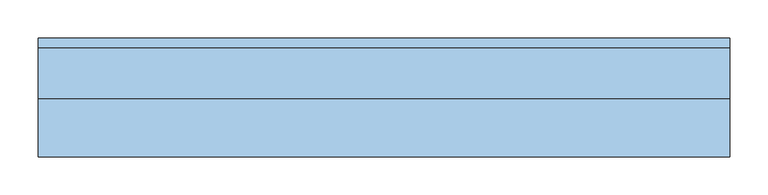
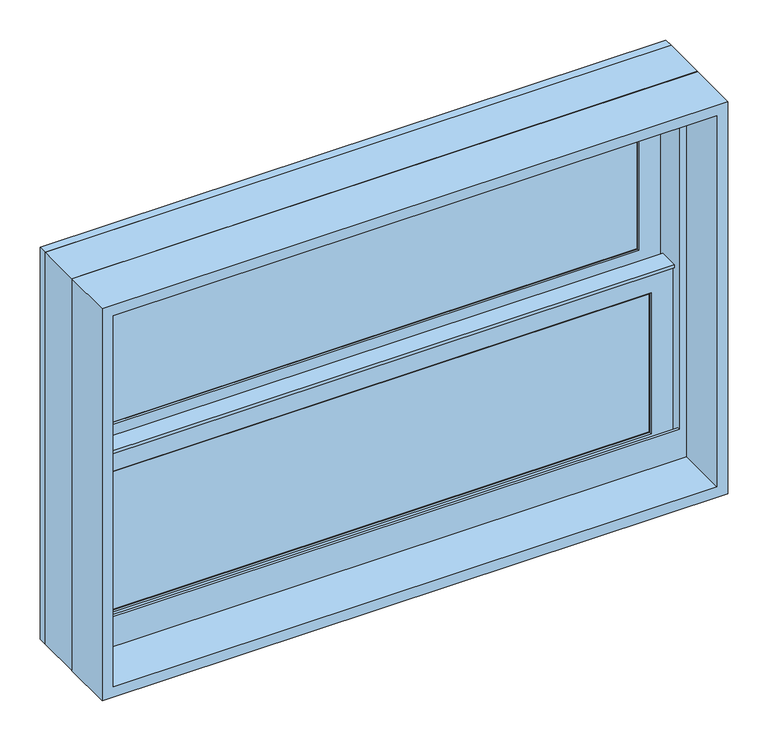
"""IFC4 building model written with IfcOpenShell, lengths in millimetres: window geometry, Window-Double_Hung-Marvin-Essential : ESDH3020."""

from ifc_helpers import new_model, si_unit, frame, origin, place, context, project, spatial, polyline, outline, extrude, faceted_brep, source, transform, mapped, element, save


def window_0800c113(model_context):
    return source(origin(), model_context, "Body", "SolidModel", [
        extrude(outline(polyline([(140.7583333, 20.6375), (140.7583333, 15.875), (121.7083333, 15.875), (121.7083333, 20.6375), (140.7583333, 20.6375)])), frame((0.0, 0.0, 1898.65), z_axis=(0.0, 0.0, 1.0), x_axis=(1.0, 0.0, 0.0)), (0.0, 0.0, 1.0), 222.25),
        extrude(outline(polyline([(-121.7083333, 20.6375), (-121.7083333, 15.875), (-140.7583333, 15.875), (-140.7583333, 20.6375), (-121.7083333, 20.6375)])), frame((0.0, 0.0, 1898.65), z_axis=(0.0, 0.0, 1.0), x_axis=(1.0, 0.0, 0.0)), (0.0, 0.0, 1.0), 222.25),
        extrude(outline(polyline([(393.7, 20.6375), (393.7, 15.875), (-393.7, 15.875), (-393.7, 20.6375), (393.7, 20.6375)])), frame((0.0, 0.0, 2000.25), z_axis=(0.0, 0.0, 1.0), x_axis=(1.0, 0.0, 0.0)), (0.0, 0.0, 1.0), 19.05),
        extrude(outline(polyline([(-140.7583333, 46.83125), (-140.7583333, 51.59375), (-121.7083333, 51.59375), (-121.7083333, 46.83125), (-140.7583333, 46.83125)])), frame((0.0, 0.0, 2159.0), z_axis=(0.0, 0.0, 1.0), x_axis=(1.0, 0.0, 0.0)), (0.0, 0.0, 1.0), 222.25),
        extrude(outline(polyline([(121.7083333, 46.83125), (121.7083333, 51.59375), (140.7583333, 51.59375), (140.7583333, 46.83125), (121.7083333, 46.83125)])), frame((0.0, 0.0, 2159.0), z_axis=(0.0, 0.0, 1.0), x_axis=(1.0, 0.0, 0.0)), (0.0, 0.0, 1.0), 222.25),
        extrude(outline(polyline([(-393.7, 46.83125), (-393.7, 51.59375), (393.7, 51.59375), (393.7, 46.83125), (-393.7, 46.83125)])), frame((0.0, 0.0, 2260.6), z_axis=(0.0, 0.0, 1.0), x_axis=(1.0, 0.0, 0.0)), (0.0, 0.0, 1.0), 19.05),
        extrude(outline(polyline([(140.7583333, 20.6375), (121.7083333, 20.6375), (121.7083333, 25.4), (140.7583333, 25.4), (140.7583333, 20.6375)])), frame((0.0, 0.0, 1898.65), z_axis=(0.0, 0.0, 1.0), x_axis=(1.0, 0.0, 0.0)), (0.0, 0.0, 1.0), 222.25),
        extrude(outline(polyline([(-121.7083333, 20.6375), (-140.7583333, 20.6375), (-140.7583333, 25.4), (-121.7083333, 25.4), (-121.7083333, 20.6375)])), frame((0.0, 0.0, 1898.65), z_axis=(0.0, 0.0, 1.0), x_axis=(1.0, 0.0, 0.0)), (0.0, 0.0, 1.0), 222.25),
        extrude(outline(polyline([(393.7, 20.6375), (-393.7, 20.6375), (-393.7, 25.4), (393.7, 25.4), (393.7, 20.6375)])), frame((0.0, 0.0, 2000.25), z_axis=(0.0, 0.0, 1.0), x_axis=(1.0, 0.0, 0.0)), (0.0, 0.0, 1.0), 19.05),
        extrude(outline(polyline([(-140.7583333, 56.35625), (-121.7083333, 56.35625), (-121.7083333, 51.59375), (-140.7583333, 51.59375), (-140.7583333, 56.35625)])), frame((0.0, 0.0, 2159.0), z_axis=(0.0, 0.0, 1.0), x_axis=(1.0, 0.0, 0.0)), (0.0, 0.0, 1.0), 222.25),
        extrude(outline(polyline([(121.7083333, 56.35625), (140.7583333, 56.35625), (140.7583333, 51.59375), (121.7083333, 51.59375), (121.7083333, 56.35625)])), frame((0.0, 0.0, 2159.0), z_axis=(0.0, 0.0, 1.0), x_axis=(1.0, 0.0, 0.0)), (0.0, 0.0, 1.0), 222.25),
        extrude(outline(polyline([(-393.7, 56.35625), (393.7, 56.35625), (393.7, 51.59375), (-393.7, 51.59375), (-393.7, 56.35625)])), frame((0.0, 0.0, 2260.6), z_axis=(0.0, 0.0, 1.0), x_axis=(1.0, 0.0, 0.0)), (0.0, 0.0, 1.0), 19.05),
        faceted_brep([(-420.6875, 5.6780605, 2150.9351748), (-420.6875, 5.6780605, 2146.3), (420.6875, 5.6780605, 2146.3), (420.6875, 5.6780605, 2150.9351748), (-420.6875, 34.8118605, 2150.9351748), (420.6875, 34.8118605, 2150.9351748), (420.6875, 34.8118605, 2146.3), (-420.6875, 34.8118605, 2146.3), (-420.6875, 30.1625, 2146.3), (-420.6875, 30.1625, 1871.6625), (-420.6875, 8.9241104, 1871.6625), (-420.6875, 8.9241104, 2146.3), (420.6875, 8.9241104, 2146.3), (420.6875, 30.1625, 2146.3), (420.6875, 8.9241104, 1871.6625), (420.6875, 30.1625, 1871.6625), (-404.8034752, 11.90625, 2132.0034752), (-404.8034752, 30.1625, 2132.0034752), (404.8034752, 30.1625, 2132.0034752), (404.8034752, 11.90625, 2132.0034752), (-388.14375, 10.4662439, 2115.34375), (-388.14375, 11.90625, 2115.34375), (388.14375, 11.90625, 2115.34375), (388.14375, 10.4662439, 2115.34375), (389.6858834, 8.9241104, 2116.8858834), (-389.6858834, 8.9241104, 2116.8858834), (404.8034752, 30.1625, 1887.5465248), (404.8034752, 11.90625, 1887.5465248), (388.14375, 11.90625, 1904.20625), (388.14375, 10.4662439, 1904.20625), (389.6858834, 8.9241104, 1902.6641166), (-404.8034752, 30.1625, 1887.5465248), (-404.8034752, 11.90625, 1887.5465248), (-388.14375, 11.90625, 1904.20625), (-388.14375, 10.4662439, 1904.20625), (-389.6858834, 8.9241104, 1902.6641166)], [[[0, 1, 2, 3]], [[4, 5, 6, 7]], [[1, 0, 4, 7, 8, 9, 10, 11]], [[2, 1, 11, 12]], [[7, 6, 13, 8]], [[3, 2, 12, 14, 15, 13, 6, 5]], [[0, 3, 5, 4]], [[16, 17, 18, 19]], [[20, 21, 22, 23]], [[20, 23, 24, 25]], [[19, 18, 26, 27]], [[23, 22, 28, 29]], [[24, 23, 29, 30]], [[27, 26, 31, 32]], [[29, 28, 33, 34]], [[30, 29, 34, 35]], [[15, 14, 10, 9]], [[15, 9, 8, 13], [18, 17, 31, 26]], [[17, 16, 32, 31]], [[16, 19, 27, 32], [22, 21, 33, 28]], [[21, 20, 34, 33]], [[20, 25, 35, 34]], [[10, 14, 12, 11], [25, 24, 30, 35]]]),
        extrude(outline(polyline([(38.5955581, 2132.0125), (33.5778968, 2132.0125), (33.5778968, 2133.6), (39.9405976, 2133.6), (39.9405976, 2132.0125), (61.515625, 2132.0125), (47.6307501, 2128.6975159), (38.5955581, 2128.6975159), (38.5955581, 2132.0125)])), frame((-420.6875, 0.0, 0.0), z_axis=(1.0, 0.0, 0.0), x_axis=(0.0, 1.0, 0.0)), (0.0, 0.0, 1.0), 841.375),
        faceted_brep([(450.85, 0.0, 1841.5), (450.85, 0.0, 2438.4), (-450.85, 0.0, 2438.4), (-450.85, 0.0, 1841.5), (424.65625, 0.0, 1902.61875), (-424.65625, 0.0, 1902.61875), (-424.65625, 0.0, 2412.20625), (424.65625, 0.0, 2412.20625), (424.65625, 3.96875, 1841.5), (-424.65625, 3.96875, 1841.5), (-424.65625, 3.96875, 1902.61875), (424.65625, 3.96875, 1902.61875), (-450.85, 65.6828125, 1841.5), (-424.65625, 65.6828125, 1841.5), (424.65625, 65.6828125, 1841.5), (450.85, 65.6828125, 1841.5), (-450.85, 65.6828125, 2438.4), (450.85, 65.6828125, 2438.4), (424.65625, 65.6828125, 2412.20625), (-424.65625, 65.6828125, 2412.20625)], [[[0, 1, 2, 3], [4, 5, 6, 7]], [[8, 9, 10, 11]], [[5, 4, 11, 10]], [[0, 3, 12, 13, 9, 8, 14, 15]], [[13, 12, 16, 17, 15, 14, 18, 19]], [[13, 19, 6, 5, 10, 9]], [[7, 6, 19, 18]], [[18, 14, 8, 11, 4, 7]], [[1, 0, 15, 17]], [[2, 1, 17, 16]], [[3, 2, 16, 12]]]),
        faceted_brep([(424.65625, 30.1625, 2139.95), (423.06875, 30.1625, 2139.95), (423.06875, 30.1625, 1865.8544613), (424.65625, 30.1625, 1865.8544613), (-423.06875, 30.1625, 2139.95), (-424.65625, 30.1625, 2139.95), (-424.65625, 30.1625, 1865.8544613), (-423.06875, 30.1625, 1865.8544613), (423.06875, 63.5, 2139.95), (424.65625, 63.5, 2139.95), (424.65625, 63.5, 1859.3743077), (423.06875, 63.5, 1859.3743077), (-424.65625, 63.5, 2139.95), (-423.06875, 63.5, 2139.95), (-423.06875, 63.5, 1859.3743077), (-424.65625, 63.5, 1859.3743077), (435.9108932, 3.96875, 1870.9460105), (435.9108932, 3.96875, 1841.5), (435.9108932, 65.6828125, 1841.5), (435.9108932, 65.6828125, 1858.950012), (-435.9108932, 3.96875, 1841.5), (-435.9108932, 3.96875, 1870.9460105), (-435.9108932, 65.6828125, 1858.950012), (-435.9108932, 65.6828125, 1841.5), (435.9108932, 78.58125, 1856.4428097), (-435.9108932, 78.58125, 1856.4428097), (-433.8971252, 68.2348864, 1858.4539391), (-415.93135, 68.2348864, 1858.4539391), (-415.93135, 65.6828125, 1858.950012), (415.93135, 65.6828125, 1858.950012), (415.93135, 68.2348864, 1858.4539391), (433.8971252, 68.2348864, 1858.4539391), (-450.85, 65.6828125, 1841.5), (-450.85, 78.5948249, 1841.5), (450.85, 78.5948249, 1841.5), (450.85, 65.6828125, 1841.5), (-450.85, 78.58125, 2438.4), (450.85, 78.58125, 2438.4), (435.9108932, 78.58125, 2423.4608932), (-435.9108932, 78.58125, 2423.4608932), (-450.85, 65.6828125, 2438.4), (-433.8971252, 68.2348864, 2421.4471252), (433.8971252, 68.2348864, 2421.4471252), (415.93135, 68.2348864, 2403.48135), (-415.93135, 68.2348864, 2403.48135), (-415.93135, 65.6828125, 2403.48135), (415.93135, 65.6828125, 2403.48135), (450.85, 65.6828125, 2438.4)], [[[0, 1, 2, 3]], [[4, 5, 6, 7]], [[8, 9, 10, 11]], [[12, 13, 14, 15]], [[1, 8, 11, 2]], [[9, 0, 3, 10]], [[1, 0, 9, 8]], [[5, 4, 13, 12]], [[5, 12, 15, 6]], [[13, 4, 7, 14]], [[16, 17, 18, 19]], [[20, 21, 22, 23]], [[24, 25, 26, 27, 28, 22, 21, 16, 19, 29, 30, 31], [3, 2, 11, 10], [7, 6, 15, 14]], [[17, 16, 21, 20]], [[17, 20, 23, 32, 33, 34, 35, 18]], [[34, 33, 36, 37], [25, 24, 38, 39]], [[33, 32, 40, 36]], [[39, 41, 26, 25]], [[41, 42, 31, 30, 43, 44, 27, 26]], [[44, 45, 28, 27]], [[40, 32, 23, 22, 28, 45, 46, 29, 19, 18, 35, 47]], [[36, 40, 47, 37]], [[39, 38, 42, 41]], [[44, 43, 46, 45]], [[34, 37, 47, 35]], [[42, 38, 24, 31]], [[46, 43, 30, 29]]]),
        extrude(outline(polyline([(400.84375, 11.90625), (-400.84375, 11.90625), (-400.84375, 15.08125), (400.84375, 15.08125), (400.84375, 11.90625)])), frame((0.0, 0.0, 1891.50625), z_axis=(0.0, 0.0, 1.0), x_axis=(1.0, 0.0, 0.0)), (0.0, 0.0, 1.0), 236.5375),
        extrude(outline(polyline([(400.84375, 42.8625), (-400.84375, 42.8625), (-400.84375, 46.0375), (400.84375, 46.0375), (400.84375, 42.8625)])), frame((0.0, 0.0, 2151.85625), z_axis=(0.0, 0.0, 1.0), x_axis=(1.0, 0.0, 0.0)), (0.0, 0.0, 1.0), 236.5375),
        faceted_brep([(-388.14375, 31.194477, 2115.34375), (-389.6858834, 32.7366104, 2116.8858834), (389.6858834, 32.7366104, 2116.8858834), (388.14375, 31.194477, 2115.34375), (-388.14375, 30.1625, 2115.34375), (388.14375, 30.1625, 2115.34375), (-420.6875, 32.7366104, 2147.8875), (-420.6875, 30.1625, 2147.8875), (420.6875, 30.1625, 2147.8875), (420.6875, 32.7366104, 2147.8875), (389.6858834, 32.7366104, 1902.6641166), (388.14375, 31.194477, 1904.20625), (388.14375, 30.1625, 1904.20625), (420.6875, 30.1625, 1871.6625), (420.6875, 32.7366104, 1871.6625), (-389.6858834, 32.7366104, 1902.6641166), (-388.14375, 31.194477, 1904.20625), (-388.14375, 30.1625, 1904.20625), (-420.6875, 30.1625, 1871.6625), (-420.6875, 32.7366104, 1871.6625)], [[[0, 1, 2, 3]], [[4, 0, 3, 5]], [[6, 7, 8, 9]], [[3, 2, 10, 11]], [[5, 3, 11, 12]], [[9, 8, 13, 14]], [[11, 10, 15, 16]], [[12, 11, 16, 17]], [[14, 13, 18, 19]], [[9, 14, 19, 6], [1, 15, 10, 2]], [[16, 15, 1, 0]], [[17, 16, 0, 4]], [[7, 18, 13, 8], [5, 12, 17, 4]], [[19, 18, 7, 6]]]),
        faceted_brep([(-404.8034752, 42.8625, 2392.3534752), (-404.8034752, 61.11875, 2392.3534752), (404.8034752, 61.11875, 2392.3534752), (404.8034752, 42.8625, 2392.3534752), (-388.14375, 41.4224939, 2375.69375), (-388.14375, 42.8625, 2375.69375), (388.14375, 42.8625, 2375.69375), (388.14375, 41.4224939, 2375.69375), (-389.6858834, 39.8803604, 2377.2358834), (389.6858834, 39.8803604, 2377.2358834), (-420.6875, 61.11875, 2408.2375), (-420.6875, 39.8803604, 2408.2375), (420.6875, 39.8803604, 2408.2375), (420.6875, 61.11875, 2408.2375), (404.8034752, 61.11875, 2147.8965248), (404.8034752, 42.8625, 2147.8965248), (388.14375, 42.8625, 2164.55625), (388.14375, 41.4224939, 2164.55625), (389.6858834, 39.8803604, 2163.0141166), (420.6875, 39.8803604, 2132.0125), (420.6875, 61.11875, 2132.0125), (-404.8034752, 61.11875, 2147.8965248), (-404.8034752, 42.8625, 2147.8965248), (-388.14375, 42.8625, 2164.55625), (-388.14375, 41.4224939, 2164.55625), (-389.6858834, 39.8803604, 2163.0141166), (-420.6875, 39.8803604, 2132.0125), (-420.6875, 61.11875, 2132.0125)], [[[0, 1, 2, 3]], [[4, 5, 6, 7]], [[8, 4, 7, 9]], [[10, 11, 12, 13]], [[3, 2, 14, 15]], [[7, 6, 16, 17]], [[9, 7, 17, 18]], [[13, 12, 19, 20]], [[15, 14, 21, 22]], [[17, 16, 23, 24]], [[18, 17, 24, 25]], [[20, 19, 26, 27]], [[13, 20, 27, 10], [1, 21, 14, 2]], [[22, 21, 1, 0]], [[3, 15, 22, 0], [5, 23, 16, 6]], [[24, 23, 5, 4]], [[25, 24, 4, 8]], [[11, 26, 19, 12], [9, 18, 25, 8]], [[27, 26, 11, 10]]]),
        faceted_brep([(-420.6875, 61.11875, 2132.0125), (-420.6875, 63.6928604, 2132.0125), (420.6875, 63.6928604, 2132.0125), (420.6875, 61.11875, 2132.0125), (-388.14375, 62.150727, 2164.55625), (-388.14375, 61.11875, 2164.55625), (388.14375, 61.11875, 2164.55625), (388.14375, 62.150727, 2164.55625), (-389.6858834, 63.6928604, 2163.0141166), (389.6858834, 63.6928604, 2163.0141166), (420.6875, 63.6928604, 2408.2375), (420.6875, 61.11875, 2408.2375), (388.14375, 61.11875, 2375.69375), (388.14375, 62.150727, 2375.69375), (389.6858834, 63.6928604, 2377.2358834), (-420.6875, 63.6928604, 2408.2375), (-420.6875, 61.11875, 2408.2375), (-388.14375, 61.11875, 2375.69375), (-388.14375, 62.150727, 2375.69375), (-389.6858834, 63.6928604, 2377.2358834)], [[[0, 1, 2, 3]], [[4, 5, 6, 7]], [[8, 4, 7, 9]], [[3, 2, 10, 11]], [[7, 6, 12, 13]], [[9, 7, 13, 14]], [[11, 10, 15, 16]], [[13, 12, 17, 18]], [[14, 13, 18, 19]], [[16, 15, 1, 0]], [[3, 11, 16, 0], [5, 17, 12, 6]], [[18, 17, 5, 4]], [[19, 18, 4, 8]], [[1, 15, 10, 2], [9, 14, 19, 8]]]),
        extrude(outline(polyline([(400.84375, 26.19375), (-400.84375, 26.19375), (-400.84375, 30.1625), (400.84375, 30.1625), (400.84375, 26.19375)])), frame((0.0, 0.0, 1891.50625), z_axis=(0.0, 0.0, 1.0), x_axis=(1.0, 0.0, 0.0)), (0.0, 0.0, 1.0), 236.5375),
        extrude(outline(polyline([(400.84375, 57.15), (-400.84375, 57.15), (-400.84375, 61.11875), (400.84375, 61.11875), (400.84375, 57.15)])), frame((0.0, 0.0, 2151.85625), z_axis=(0.0, 0.0, 1.0), x_axis=(1.0, 0.0, 0.0)), (0.0, 0.0, 1.0), 236.5375),
        extrude(outline(polyline([(2438.4, 450.85), (2438.4, -450.85), (1841.5, -450.85), (1841.5, 450.85), (2438.4, 450.85)]), holes=[polyline([(2422.525, 434.975), (1857.375, 434.975), (1857.375, -434.975), (2422.525, -434.975), (2422.525, 434.975)])]), frame((0.0, -76.2, 0.0), z_axis=(0.0, 1.0, 0.0), x_axis=(0.0, 0.0, 1.0)), (0.0, 0.0, 1.0), 75.40625),
    ])


if __name__ == "__main__":
    model = new_model("IFC4")
    model_context = context("Model", 3, world=origin())
    ifc_project = project(units=[si_unit("LENGTHUNIT", "METRE", prefix="MILLI")], contexts=[model_context])
    site = spatial("IfcSite", under=ifc_project)
    building = spatial("IfcBuilding", under=site)
    placement = place(None, origin())
    window_shape = window_0800c113(model_context)
    element("IfcWindow", 1, ObjectType="Window-Double_Hung-Marvin-Essential : ESDH3020", at=placement, inside=building, context=model_context, shape_type="MappedRepresentation", body=[
        mapped(window_shape, transform((0.0, 0.0, 0.0), x_axis=(1.0, 0.0, 0.0), y_axis=(0.0, 1.0, 0.0), z_axis=(0.0, 0.0, 1.0))),
    ])
    save(model, "model.ifc")

# Revit data of these elements
# Type "Window-Double_Hung-Marvin-Essential : ESDH3020"
#   Type Mark = "23"
#   Window Type = "Essential Double Hung"
#   Product data url = "https://bimobject.com/marvin-windows-and-doors/product/marvin-dhwau"
#   Product Guid = "c4a96547-874c-4385-91dc-a058adc19d98"
#   Frame = "All Ultrex"
#   Egress Window = "No"
#   URL = "www.marvin.com"
#   Model = "ESDH3020"
#   Manufacturer = "Marvin Windows and Doors"
#   Label Egress = ""
#   Glass Type = "IG Low E II with Argon"
#   Design Pressure = "DP50"
#   Description = "3624 DBHG"
#   Analytic Construction = "<None>"
#   Prairie Corner Width = 0' - 4"
#   Prairie Corner Height = 0' - 4"
#   Egress Width = 2' - 8 9/16"
#   Egress Height = 0' - 7 27/128"
#   Rough Width = 3' - 0"
#   Rough Height = 2' - 0"
#   Nominal Width = 3' - 0"
#   Nominal Height = 2' - 0"
#   Inset to Installation Flange [instance default] = 0' - 1"
#   Height = 1' - 11 1/2"
#   Egress Area = 1.6306 SF
#   Default Head Height = 8' - 0"
#   Width = 2' - 11 1/2"
#   Daylight Area = 3.52848 SF
#   DLO Width = 2' - 6 9/16"
#   DLO Height = 0' - 8 5/16"
#   Muntins Top Sash = yes
#   Lites Wide Top Sash = 3
#   Lites Wide Bottom Sash = 3
#   Lites High Top Sash = 2
#   Lites High Bottom Sash = 2
#   Lite Cut Prairie 9 = no
#   Lite Cut HV Grid = yes
#   Muntins Bottom Sash = yes
#   Label Visibility = no
#   Jamb Extension Visibility = yes
#   Edition number = 1
#   Interior Material = Ultrex-Marvin-Stonewhite
#   Glazing Material = Glass-Marvin-IG Low E II with Argon
#   Cladding Material = Ultrex-Marvin-Pebblegray
#   Wall Closure = (empty or 0)
#   Assembly Code = ""
# Element 1 (IfcWindow, "Window-Double_Hung-Marvin-Essential : ESDH3020")
#   Materials on its faces: "Ultrex-Marvin-Pebblegray", "Ultrex-Marvin-Stonewhite", "Glass-Marvin-IG Low E II with Argon"
# Materials
#   "Ultrex-Marvin-Stonewhite": class "Paint", colour RGB 250 251 245, transparency 0
#   "Glass-Marvin-IG Low E II with Argon": class "Glass", colour RGB 0 128 192, transparency 0.85
#   "Ultrex-Marvin-Pebblegray": class "Paint", colour RGB 189 185 173, transparency 0
